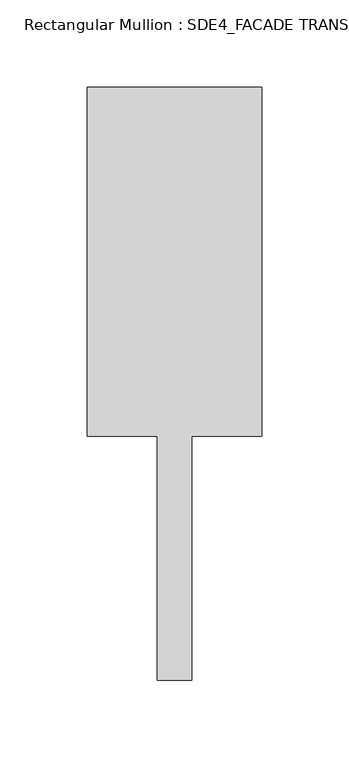
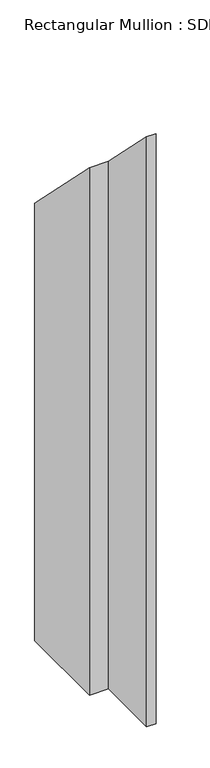
"""IFC4 building model written with IfcOpenShell, lengths in millimetres: member geometry, Rectangular Mullion : SDE4_FACADE TRANSOM TYPE 1."""

import ifcopenshell
import ifcopenshell.guid

model = None  # the IFC model being written
_history = None  # IfcOwnerHistory: only IFC2X3 demands one
_inside = {}  # id of a spatial element -> (the spatial element, [elements in it])
_under = {}  # id of a project, library or spatial element -> (it, [spatial elements below it])
_declared = {}  # id of a project -> (the project, [libraries it declares])
_typed = {}  # id of a type object -> (the type object, [elements of that type])
_made_of = {}  # id of a material, layer set ... -> (it, [elements and type objects made of it])


def new_model(schema):
    """Start an empty IFC model of exactly this schema.

    Asked for "IFC4X3", IfcOpenShell would pick the latest addendum, in which some entities
    have other attributes; the version numbers below select the first issue.
    IFC2X3 requires an IfcOwnerHistory on every rooted entity: one is made here for all.
    """
    global model, _history
    if schema == "IFC4X3":
        model = ifcopenshell.file(schema_version=(4, 3, 0, 0))
    else:
        model = ifcopenshell.file(schema=schema)
    _inside.clear()
    _under.clear()
    _declared.clear()
    _typed.clear()
    _made_of.clear()
    _history = None
    if model.schema == "IFC2X3":
        org = make("IfcOrganization", Name="unknown")
        user = make(
            "IfcPersonAndOrganization",
            ThePerson=make("IfcPerson", FamilyName="unknown"),
            TheOrganization=org,
        )
        app = make(
            "IfcApplication",
            ApplicationDeveloper=org,
            Version="unknown",
            ApplicationFullName="unknown",
            ApplicationIdentifier="unknown",
        )
        _history = make(
            "IfcOwnerHistory",
            OwningUser=user,
            OwningApplication=app,
            ChangeAction="ADDED",
            CreationDate=0,
        )
    return model


def make(cls, **values):
    """One entity of the class cls with the attributes given. An attribute that is None is left unset."""
    return model.create_entity(
        cls, **{name: value for name, value in values.items() if value is not None}
    )


def rooted(cls, **values):
    """An entity with a GlobalId (a new one), such as an element, a storey or a relation."""
    return make(cls, GlobalId=ifcopenshell.guid.new(), OwnerHistory=_history, **values)


def si_unit(unit_type, name, prefix=None):
    """IfcSIUnit, for example si_unit("LENGTHUNIT", "METRE", prefix="MILLI")."""
    return make("IfcSIUnit", UnitType=unit_type, Prefix=prefix, Name=name)


def assignment(units):
    """IfcUnitAssignment: the units of a project."""
    return None if units is None else make("IfcUnitAssignment", Units=units)


def point(xyz):
    """IfcCartesianPoint."""
    return None if xyz is None else make("IfcCartesianPoint", Coordinates=xyz)


def direction(xyz):
    """IfcDirection."""
    return None if xyz is None else make("IfcDirection", DirectionRatios=xyz)


def frame(location, z_axis=None, x_axis=None):
    """IfcAxis2Placement3D, a coordinate frame: its origin and axes. An axis left out is left unset."""
    return make(
        "IfcAxis2Placement3D",
        Location=point(location),
        Axis=direction(z_axis),
        RefDirection=direction(x_axis),
    )


def origin():
    """The frame at (0, 0, 0) with its axes left unset."""
    return frame((0.0, 0.0, 0.0))


def place(relative_to, where):
    """IfcLocalPlacement: puts the frame where relative to a parent placement (None: the world)."""
    return make(
        "IfcLocalPlacement", PlacementRelTo=relative_to, RelativePlacement=where
    )


def context(
    kind, dimensions, precision=None, world=None, true_north=None, identifier=None
):
    """IfcGeometricRepresentationContext, for example the 3D "Model" context."""
    return make(
        "IfcGeometricRepresentationContext",
        ContextIdentifier=identifier,
        ContextType=kind,
        CoordinateSpaceDimension=dimensions,
        Precision=precision,
        WorldCoordinateSystem=world,
        TrueNorth=true_north,
    )


def project(units=None, contexts=None):
    """IfcProject with its units and contexts."""
    return rooted(
        "IfcProject",
        Name="project",
        RepresentationContexts=contexts,
        UnitsInContext=assignment(units),
    )


def spatial(cls, under=None, at=None, **own):
    """A site, building, storey or space (cls), placed at a placement, below another one or the project."""
    s = rooted(cls, ObjectPlacement=at, **own)
    if under is not None:
        _under.setdefault(under.id(), (under, []))[1].append(s)
    return s


def faces_of(points, faces, orient=None, outer=None):
    """IfcFace entities. A face is a list of loops; a loop is a list of indices into points, from 0.

    orient and outer hold one flag for each loop. By default every Orientation is true, the
    first loop of a face is its IfcFaceOuterBound and the others are IfcFaceBound.
    """
    made = []
    for i, loops in enumerate(faces):
        bounds = []
        for j, loop in enumerate(loops):
            is_outer = j == 0 if outer is None else outer[i][j]
            bounds.append(
                make(
                    "IfcFaceOuterBound" if is_outer else "IfcFaceBound",
                    Bound=make("IfcPolyLoop", Polygon=[points[k] for k in loop]),
                    Orientation=True if orient is None else orient[i][j],
                )
            )
        made.append(make("IfcFace", Bounds=bounds))
    return made


def faceted_brep(points, faces, orient=None, outer=None, voids=None):
    """IfcFacetedBrep: a solid bounded by flat faces; with voids (closed shells), ...WithVoids."""
    shared = [point(p) for p in points]
    hull = make("IfcClosedShell", CfsFaces=faces_of(shared, faces, orient, outer))
    if voids is None:
        return make("IfcFacetedBrep", Outer=hull)
    return make(
        "IfcFacetedBrepWithVoids",
        Outer=hull,
        Voids=[
            make(cls, CfsFaces=faces_of(shared, fs, o, b)) for cls, fs, o, b in voids
        ],
    )


def shape(context_of_items, identifier, shape_type, items):
    """IfcShapeRepresentation: the items that make up one representation, for example the "Body"."""
    return make(
        "IfcShapeRepresentation",
        ContextOfItems=context_of_items,
        RepresentationIdentifier=identifier,
        RepresentationType=shape_type,
        Items=items,
    )


def source(mapping_origin, context_of_items, identifier, shape_type, items):
    """IfcRepresentationMap: a shape defined once, which mapped items show again and again."""
    return make(
        "IfcRepresentationMap",
        MappingOrigin=mapping_origin,
        MappedRepresentation=shape(context_of_items, identifier, shape_type, items),
    )


def transform(
    local_origin,
    x_axis=None,
    y_axis=None,
    z_axis=None,
    scale=None,
    scale2=None,
    scale3=None,
    uniform=True,
):
    """IfcCartesianTransformationOperator3D, or its non-uniform kind. x_axis, y_axis, z_axis: its Axis1, 2, 3."""
    if uniform:
        return make(
            "IfcCartesianTransformationOperator3D",
            Axis1=direction(x_axis),
            Axis2=direction(y_axis),
            LocalOrigin=point(local_origin),
            Scale=scale,
            Axis3=direction(z_axis),
        )
    return make(
        "IfcCartesianTransformationOperator3DnonUniform",
        Axis1=direction(x_axis),
        Axis2=direction(y_axis),
        LocalOrigin=point(local_origin),
        Scale=scale,
        Axis3=direction(z_axis),
        Scale2=scale2,
        Scale3=scale3,
    )


def mapped(mapping_source, mapping_target):
    """IfcMappedItem: shows the shape of a source again, moved by a transform."""
    return make(
        "IfcMappedItem", MappingSource=mapping_source, MappingTarget=mapping_target
    )


def made_of(thing, what):
    """Note that an element or type object is made of a material, layer set ...; save() writes the relation."""
    if what is not None:
        _made_of.setdefault(what.id(), (what, []))[1].append(thing)
    return thing


def element(
    cls,
    number,
    at=None,
    inside=None,
    cuts=None,
    type_object=None,
    material=None,
    context=None,
    identifier="Body",
    shape_type=None,
    held_by="IfcProductDefinitionShape",
    body=None,
    shapes=None,
    **own,
):
    """One element of the class cls, such as IfcWall. Its Tag is "e" and its number.

    at: its placement. inside: the storey or other place that contains it. cuts: it is an
    opening in that element (IfcRelVoidsElement). A single representation is given by context,
    identifier, shape_type and body (its items); several are given by shapes. held_by: the class
    of the entity that holds the representations. save() writes the other relations.
    """
    e = rooted(cls, Tag="e%d" % number, ObjectPlacement=at, **own)
    if body is not None:
        shapes = [shape(context, identifier, shape_type, body)]
    if shapes is not None:
        e.Representation = make(held_by, Representations=shapes)
    if inside is not None:
        _inside.setdefault(inside.id(), (inside, []))[1].append(e)
    if cuts is not None:
        rooted(
            "IfcRelVoidsElement", RelatingBuildingElement=cuts, RelatedOpeningElement=e
        )
    if type_object is not None:
        _typed.setdefault(type_object.id(), (type_object, []))[1].append(e)
    return made_of(e, material)


def aggregate(whole, parts):
    """IfcRelAggregates: a whole, such as a stair, and the parts it consists of."""
    return rooted("IfcRelAggregates", RelatingObject=whole, RelatedObjects=parts)


def save(model, path):
    """Write the relations noted so far, then the file.

    IfcRelAggregates (storeys below a building ...), IfcRelContainedInSpatialStructure (elements
    in a storey), IfcRelDefinesByType, IfcRelAssociatesMaterial and IfcRelDeclares: one each for
    every whole, place, type object, material and project.
    """
    for whole, parts in _under.values():
        aggregate(whole, parts)
    for where, things in _inside.values():
        rooted(
            "IfcRelContainedInSpatialStructure",
            RelatedElements=things,
            RelatingStructure=where,
        )
    for kind, things in _typed.values():
        rooted("IfcRelDefinesByType", RelatedObjects=things, RelatingType=kind)
    for what, things in _made_of.values():
        rooted("IfcRelAssociatesMaterial", RelatedObjects=things, RelatingMaterial=what)
    for by, libraries in _declared.values():
        rooted("IfcRelDeclares", RelatingContext=by, RelatedDefinitions=libraries)
    model.write(path)


def rectangular_mullion_sde4_facade_transom_type_1_2e7e779c(model_context):
    return source(origin(), model_context, "Body", "Brep", [
        faceted_brep([(50.0, 132.5, -1108.75), (50.0, -67.5, -1108.75), (10.0, -67.5, -1108.75), (10.0, -207.5, -1108.75), (-10.0, -207.5, -1108.75), (-10.0, -67.5, -1108.75), (-50.0, -67.5, -1108.75), (-50.0, 132.5, -1108.75), (-50.0, 132.5, -132.5), (50.0, 132.5, -132.5), (-50.0, -67.5, 67.5), (-10.0, -67.5, 67.5), (-10.0, -207.5, 207.5), (10.0, -207.5, 207.5), (10.0, -67.5, 67.5), (50.0, -67.5, 67.5)], [[[0, 1, 2, 3, 4, 5, 6, 7]], [[8, 9, 0, 7]], [[10, 8, 7, 6]], [[11, 10, 6, 5]], [[12, 11, 5, 4]], [[13, 12, 4, 3]], [[14, 13, 3, 2]], [[15, 14, 2, 1]], [[9, 15, 1, 0]], [[9, 8, 10, 11, 12, 13, 14, 15]]]),
    ])


if __name__ == "__main__":
    model = new_model("IFC4")
    model_context = context("Model", 3, world=origin())
    ifc_project = project(units=[si_unit("LENGTHUNIT", "METRE", prefix="MILLI")], contexts=[model_context])
    site = spatial("IfcSite", under=ifc_project)
    building = spatial("IfcBuilding", under=site)
    placement = place(None, origin())
    rectangular_mullion_sde4_facade_transom_type_1_shape = rectangular_mullion_sde4_facade_transom_type_1_2e7e779c(model_context)
    element("IfcMember", 1, ObjectType="Rectangular Mullion : SDE4_FACADE TRANSOM TYPE 1", at=placement, inside=building, context=model_context, shape_type="MappedRepresentation", body=[
        mapped(rectangular_mullion_sde4_facade_transom_type_1_shape, transform((0.0, 0.0, 0.0), x_axis=(1.0, 0.0, 0.0), y_axis=(0.0, 1.0, 0.0), z_axis=(0.0, 0.0, 1.0))),
    ])
    save(model, "model.ifc")

# Revit data of these elements
# Type "Rectangular Mullion : SDE4_FACADE TRANSOM TYPE 1"
#   built-in parameter 1007322 = 1.11549 (stored number, unit not read)
#   built-in parameter 1007321 = 0.164042 (stored number, unit not read)
#   built-in parameter 1007320 = 0.164042 (stored number, unit not read)
